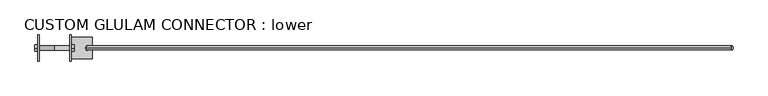
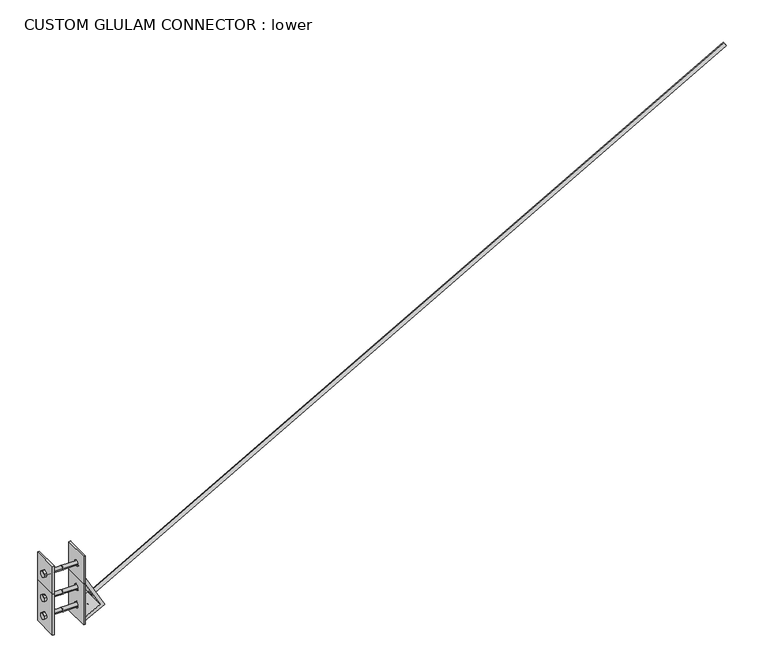
"""IFC4 building model written with IfcOpenShell, lengths in millimetres: fastener geometry, CUSTOM GLULAM CONNECTOR : lower."""

from ifc_helpers import new_model, si_unit, point, frame, frame_2d, origin, place, context, project, spatial, polyline, circle_curve, trimmed, segment, composite_curve, outline, extrude, source, transform, mapped, element, save
from ifc_brep_helpers import plane_surface, revolved_surface, advanced_brep


def custom_glulam_connector_lower_2ef7f48c(model_context):
    return source(origin(), model_context, "Body", "SolidModel", [
        advanced_brep(
        [(-77.7875, -60.325, 211.1375), (-77.7875, -52.3875, 211.1375), (-77.7875, 60.325, 211.1375), (-77.7875, 60.325, 7.9375), (-77.7875, -52.3875, 7.9375), (-77.7875, -60.325, 7.9375), (-77.7875, -13.890625, 160.3375), (-77.7875, 13.890625, 160.3375), (-77.7875, -13.890625, 71.4375), (-77.7875, 13.890625, 71.4375), (-69.85, 13.890625, 160.3375), (-69.85, -13.890625, 160.3375), (-69.85, 13.890625, 71.4375), (-69.85, -13.890625, 71.4375), (-69.85, -60.325, 211.1375), (-69.85, -60.325, 7.9375), (-69.85, 60.325, 7.9375), (-69.85, 60.325, 211.1375)],
        [
            (0, 1),
            (1, 2),
            (2, 3),
            (3, 4),
            (4, 5),
            (5, 0),
            (6, 7, circle_curve(frame((-77.7875, 0.0, 160.3375), z_axis=(1.0, 0.0, 0.0), x_axis=(0.0, -1.0, 0.0)), 13.890625)),
            (7, 6, circle_curve(frame((-77.7875, 0.0, 160.3375), z_axis=(1.0, 0.0, 0.0), x_axis=(0.0, -1.0, 0.0)), 13.890625)),
            (8, 9, circle_curve(frame((-77.7875, 0.0, 71.4375), z_axis=(1.0, 0.0, 0.0), x_axis=(0.0, -1.0, 0.0)), 13.890625)),
            (9, 8, circle_curve(frame((-77.7875, 0.0, 71.4375), z_axis=(1.0, 0.0, 0.0), x_axis=(0.0, -1.0, 0.0)), 13.890625)),
            (10, 7),
            (6, 11),
            (11, 10, circle_curve(frame((-69.85, 0.0, 160.3375), z_axis=(1.0, 0.0, 0.0), x_axis=(0.0, -1.0, 0.0)), 13.890625)),
            (10, 11, circle_curve(frame((-69.85, 0.0, 160.3375), z_axis=(1.0, 0.0, 0.0), x_axis=(0.0, -1.0, 0.0)), 13.890625)),
            (9, 12),
            (12, 13, circle_curve(frame((-69.85, 0.0, 71.4375), z_axis=(1.0, 0.0, 0.0), x_axis=(0.0, -1.0, 0.0)), 13.890625)),
            (13, 8),
            (13, 12, circle_curve(frame((-69.85, 0.0, 71.4375), z_axis=(1.0, 0.0, 0.0), x_axis=(0.0, -1.0, 0.0)), 13.890625)),
            (14, 15),
            (15, 16),
            (16, 17),
            (17, 14),
            (0, 14),
            (17, 2),
            (16, 3),
            (15, 5),
        ],
        [
            plane_surface(frame((-77.7875, 60.325, 211.1375), z_axis=(-1.0, 0.0, 0.0), x_axis=(0.0, 1.0, 0.0))),
            revolved_surface(polyline([(-77.7875, -13.890625, 160.3375), (-69.85, -13.890625, 160.3375)]), (-69.85, 0.0, 160.3375), (-1.0, 0.0, 0.0)),
            revolved_surface(polyline([(-77.7875, -13.890625, 71.4375), (-69.85, -13.890625, 71.4375)]), (-69.85, 0.0, 71.4375), (-1.0, 0.0, 0.0)),
            plane_surface(frame((-69.85, 60.325, 211.1375), z_axis=(1.0, 0.0, 0.0), x_axis=(0.0, -1.0, 0.0))),
            plane_surface(frame((-77.7875, -60.325, 211.1375), z_axis=(0.0, 0.0, 1.0), x_axis=(1.0, 0.0, 0.0))),
            plane_surface(frame((-77.7875, 60.325, 211.1375), z_axis=(0.0, 1.0, 0.0), x_axis=(1.0, 0.0, 0.0))),
            plane_surface(frame((-77.7875, 60.325, 7.9375), z_axis=(0.0, 0.0, -1.0), x_axis=(1.0, 0.0, 0.0))),
            plane_surface(frame((-77.7875, -60.325, 7.9375), z_axis=(0.0, -1.0, 0.0), x_axis=(1.0, 0.0, 0.0))),
        ],
        [
            (0, [[1, 2, 3, 4, 5, 6], [7, 8], [9, 10]]),
            (1, [[11, -7, 12, 13]]),
            (1, [[-11, 14, -12, -8]]),
            (2, [[15, 16, 17, -10]]),
            (2, [[-15, -9, -17, 18]]),
            (3, [[19, 20, 21, 22], [-13, -14], [-18, -16]]),
            (4, [[-2, -1, 23, -22, 24]]),
            (5, [[-3, -24, -21, 25]]),
            (6, [[-5, -4, -25, -20, 26]]),
            (7, [[-6, -26, -19, -23]]),
        ],
    ),
        extrude(outline(polyline([(14.2875, 168.586392), (14.2875, 152.088608), (0.0, 143.8397161), (-14.2875, 152.088608), (-14.2875, 168.586392), (0.0, 176.8352839), (14.2875, 168.586392)])), frame((-90.4875, 0.0, 0.0), z_axis=(1.0, 0.0, 0.0), x_axis=(0.0, 1.0, 0.0)), (0.0, 0.0, 1.0), 12.7),
        extrude(outline(composite_curve([segment(trimmed(circle_curve(frame_2d((0.0, 160.3375)), 9.525), [point((9.525, 160.3375))], [point((-9.525, 160.3375))], False, "CARTESIAN"), True, "CONTINUOUS"), segment(trimmed(circle_curve(frame_2d((0.0, 160.3375)), 9.525), [point((-9.525, 160.3375))], [point((9.525, 160.3375))], False, "CARTESIAN"), True, "CONTINUOUS")], self_intersect=False)), frame((-77.7875, 0.0, 0.0), z_axis=(1.0, 0.0, 0.0), x_axis=(0.0, 1.0, 0.0)), (0.0, 0.0, 1.0), 76.2),
        extrude(outline(polyline([(14.2875, 79.686392), (14.2875, 63.188608), (0.0, 54.9397161), (-14.2875, 63.188608), (-14.2875, 79.686392), (0.0, 87.9352839), (14.2875, 79.686392)])), frame((-90.4875, 0.0, 0.0), z_axis=(1.0, 0.0, 0.0), x_axis=(0.0, 1.0, 0.0)), (0.0, 0.0, 1.0), 12.7),
        extrude(outline(composite_curve([segment(trimmed(circle_curve(frame_2d((0.0, 71.4375)), 9.525), [point((9.525, 71.4375))], [point((-9.525, 71.4375))], False, "CARTESIAN"), True, "CONTINUOUS"), segment(trimmed(circle_curve(frame_2d((0.0, 71.4375)), 9.525), [point((-9.525, 71.4375))], [point((9.525, 71.4375))], False, "CARTESIAN"), True, "CONTINUOUS")], self_intersect=False)), frame((-77.7875, 0.0, 0.0), z_axis=(1.0, 0.0, 0.0), x_axis=(0.0, 1.0, 0.0)), (0.0, 0.0, 1.0), 76.2),
        extrude(outline(polyline([(14.2875, 168.586392), (14.2875, 152.088608), (0.0, 143.8397161), (-14.2875, 152.088608), (-14.2875, 168.586392), (0.0, 176.8352839), (14.2875, 168.586392)])), frame((-90.4875, 0.0, 0.0), z_axis=(1.0, 0.0, 0.0), x_axis=(0.0, 1.0, 0.0)), (0.0, 0.0, 1.0), 12.7),
        extrude(outline(composite_curve([segment(trimmed(circle_curve(frame_2d((0.0, 160.3375)), 9.525), [point((9.525, 160.3375))], [point((-9.525, 160.3375))], False, "CARTESIAN"), True, "CONTINUOUS"), segment(trimmed(circle_curve(frame_2d((0.0, 160.3375)), 9.525), [point((-9.525, 160.3375))], [point((9.525, 160.3375))], False, "CARTESIAN"), True, "CONTINUOUS")], self_intersect=False)), frame((-77.7875, 0.0, 0.0), z_axis=(1.0, 0.0, 0.0), x_axis=(0.0, 1.0, 0.0)), (0.0, 0.0, 1.0), 76.2),
        advanced_brep(
        [(77.7875, -60.325, 211.1375), (77.7875, -60.325, 7.9375), (77.7875, -52.3875, 7.9375), (77.7875, 60.325, 7.9375), (77.7875, 60.325, 211.1375), (77.7875, -52.3875, 211.1375), (77.7875, -13.890625, 71.4375), (77.7875, 13.890625, 71.4375), (77.7875, -13.890625, 160.3375), (77.7875, 13.890625, 160.3375), (69.85, 13.890625, 160.3375), (69.85, -13.890625, 160.3375), (69.85, -13.890625, 71.4375), (69.85, 13.890625, 71.4375), (69.85, -60.325, 211.1375), (69.85, 60.325, 211.1375), (69.85, 60.325, 7.9375), (69.85, -60.325, 7.9375)],
        [
            (0, 1),
            (1, 2),
            (2, 3),
            (3, 4),
            (4, 5),
            (5, 0),
            (6, 7, circle_curve(frame((77.7875, 0.0, 71.4375), z_axis=(-1.0, 0.0, 0.0), x_axis=(0.0, -1.0, 0.0)), 13.890625)),
            (7, 6, circle_curve(frame((77.7875, 0.0, 71.4375), z_axis=(-1.0, 0.0, 0.0), x_axis=(0.0, -1.0, 0.0)), 13.890625)),
            (8, 9, circle_curve(frame((77.7875, 0.0, 160.3375), z_axis=(-1.0, 0.0, 0.0), x_axis=(0.0, -1.0, 0.0)), 13.890625)),
            (9, 8, circle_curve(frame((77.7875, 0.0, 160.3375), z_axis=(-1.0, 0.0, 0.0), x_axis=(0.0, -1.0, 0.0)), 13.890625)),
            (10, 11, circle_curve(frame((69.85, 0.0, 160.3375), z_axis=(-1.0, 0.0, 0.0), x_axis=(0.0, -1.0, 0.0)), 13.890625)),
            (11, 8),
            (9, 10),
            (11, 10, circle_curve(frame((69.85, 0.0, 160.3375), z_axis=(-1.0, 0.0, 0.0), x_axis=(0.0, -1.0, 0.0)), 13.890625)),
            (6, 12),
            (12, 13, circle_curve(frame((69.85, 0.0, 71.4375), z_axis=(-1.0, 0.0, 0.0), x_axis=(0.0, -1.0, 0.0)), 13.890625)),
            (13, 7),
            (13, 12, circle_curve(frame((69.85, 0.0, 71.4375), z_axis=(-1.0, 0.0, 0.0), x_axis=(0.0, -1.0, 0.0)), 13.890625)),
            (14, 15),
            (15, 16),
            (16, 17),
            (17, 14),
            (4, 15),
            (14, 0),
            (3, 16),
            (1, 17),
        ],
        [
            plane_surface(frame((77.7875, 60.325, 211.1375), z_axis=(1.0, 0.0, 0.0), x_axis=(0.0, 1.0, 0.0))),
            revolved_surface(polyline([(77.7875, -13.890625, 160.3375), (69.85, -13.890625, 160.3375)]), (69.85, 0.0, 160.3375), (1.0, 0.0, 0.0)),
            revolved_surface(polyline([(77.7875, -13.890625, 71.4375), (69.85, -13.890625, 71.4375)]), (69.85, 0.0, 71.4375), (1.0, 0.0, 0.0)),
            plane_surface(frame((69.85, 60.325, 211.1375), z_axis=(-1.0, 0.0, 0.0), x_axis=(0.0, -1.0, 0.0))),
            plane_surface(frame((77.7875, -60.325, 211.1375), z_axis=(0.0, 0.0, 1.0), x_axis=(-1.0, 0.0, 0.0))),
            plane_surface(frame((77.7875, 60.325, 211.1375), z_axis=(0.0, 1.0, 0.0), x_axis=(-1.0, 0.0, 0.0))),
            plane_surface(frame((77.7875, 60.325, 7.9375), z_axis=(0.0, 0.0, -1.0), x_axis=(-1.0, 0.0, 0.0))),
            plane_surface(frame((77.7875, -60.325, 7.9375), z_axis=(0.0, -1.0, 0.0), x_axis=(-1.0, 0.0, 0.0))),
        ],
        [
            (0, [[1, 2, 3, 4, 5, 6], [7, 8], [9, 10]]),
            (1, [[11, 12, -10, 13]]),
            (1, [[-9, -12, 14, -13]]),
            (2, [[-7, 15, 16, 17]]),
            (2, [[18, -15, -8, -17]]),
            (3, [[19, 20, 21, 22], [-16, -18], [-14, -11]]),
            (4, [[23, -19, 24, -6, -5]]),
            (5, [[25, -20, -23, -4]]),
            (6, [[26, -21, -25, -3, -2]]),
            (7, [[-24, -22, -26, -1]]),
        ],
    ),
        extrude(outline(polyline([(14.2875, 168.586392), (14.2875, 152.088608), (0.0, 143.8397161), (-14.2875, 152.088608), (-14.2875, 168.586392), (0.0, 176.8352839), (14.2875, 168.586392)])), frame((77.7875, 0.0, 0.0), z_axis=(1.0, 0.0, 0.0), x_axis=(0.0, 1.0, 0.0)), (0.0, 0.0, 1.0), 12.7),
        extrude(outline(composite_curve([segment(trimmed(circle_curve(frame_2d((0.0, 160.3375)), 9.525), [point((9.525, 160.3375))], [point((-9.525, 160.3375))], False, "CARTESIAN"), True, "CONTINUOUS"), segment(trimmed(circle_curve(frame_2d((0.0, 160.3375)), 9.525), [point((-9.525, 160.3375))], [point((9.525, 160.3375))], False, "CARTESIAN"), True, "CONTINUOUS")], self_intersect=False)), frame((1.5875, 0.0, 0.0), z_axis=(1.0, 0.0, 0.0), x_axis=(0.0, 1.0, 0.0)), (0.0, 0.0, 1.0), 76.2),
        extrude(outline(polyline([(14.2875, 79.686392), (14.2875, 63.188608), (0.0, 54.9397161), (-14.2875, 63.188608), (-14.2875, 79.686392), (0.0, 87.9352839), (14.2875, 79.686392)])), frame((77.7875, 0.0, 0.0), z_axis=(1.0, 0.0, 0.0), x_axis=(0.0, 1.0, 0.0)), (0.0, 0.0, 1.0), 12.7),
        extrude(outline(composite_curve([segment(trimmed(circle_curve(frame_2d((0.0, 71.4375)), 9.525), [point((9.525, 71.4375))], [point((-9.525, 71.4375))], False, "CARTESIAN"), True, "CONTINUOUS"), segment(trimmed(circle_curve(frame_2d((0.0, 71.4375)), 9.525), [point((-9.525, 71.4375))], [point((9.525, 71.4375))], False, "CARTESIAN"), True, "CONTINUOUS")], self_intersect=False)), frame((1.5875, 0.0, 0.0), z_axis=(1.0, 0.0, 0.0), x_axis=(0.0, 1.0, 0.0)), (0.0, 0.0, 1.0), 76.2),
        extrude(outline(polyline([(14.2875, 168.586392), (14.2875, 152.088608), (0.0, 143.8397161), (-14.2875, 152.088608), (-14.2875, 168.586392), (0.0, 176.8352839), (14.2875, 168.586392)])), frame((77.7875, 0.0, 0.0), z_axis=(1.0, 0.0, 0.0), x_axis=(0.0, 1.0, 0.0)), (0.0, 0.0, 1.0), 12.7),
        extrude(outline(composite_curve([segment(trimmed(circle_curve(frame_2d((0.0, 160.3375)), 9.525), [point((9.525, 160.3375))], [point((-9.525, 160.3375))], False, "CARTESIAN"), True, "CONTINUOUS"), segment(trimmed(circle_curve(frame_2d((0.0, 160.3375)), 9.525), [point((-9.525, 160.3375))], [point((9.525, 160.3375))], False, "CARTESIAN"), True, "CONTINUOUS")], self_intersect=False)), frame((1.5875, 0.0, 0.0), z_axis=(1.0, 0.0, 0.0), x_axis=(0.0, 1.0, 0.0)), (0.0, 0.0, 1.0), 76.2),
        advanced_brep(
        [(-77.7875, -60.325, 350.8375), (-77.7875, 52.3875, 350.8375), (-77.7875, 60.325, 350.8375), (-77.7875, 60.325, 211.1375), (-77.7875, 52.3875, 211.1375), (-77.7875, -60.325, 211.1375), (-77.7875, -13.890625, 280.9875), (-77.7875, 13.890625, 280.9875), (-69.85, -60.325, 350.8375), (-69.85, -60.325, 211.1375), (-69.85, 60.325, 211.1375), (-69.85, 60.325, 350.8375), (-69.85, 13.890625, 280.9875), (-69.85, -13.890625, 280.9875)],
        [
            (0, 1),
            (1, 2),
            (2, 3),
            (3, 4),
            (4, 5),
            (5, 0),
            (6, 7, circle_curve(frame((-77.7875, 0.0, 280.9875), z_axis=(1.0, 0.0, 0.0), x_axis=(0.0, -1.0, 0.0)), 13.890625)),
            (7, 6, circle_curve(frame((-77.7875, 0.0, 280.9875), z_axis=(1.0, 0.0, 0.0), x_axis=(0.0, -1.0, 0.0)), 13.890625)),
            (8, 9),
            (9, 10),
            (10, 11),
            (11, 8),
            (12, 13, circle_curve(frame((-69.85, 0.0, 280.9875), z_axis=(-1.0, 0.0, 0.0), x_axis=(0.0, -1.0, 0.0)), 13.890625)),
            (13, 12, circle_curve(frame((-69.85, 0.0, 280.9875), z_axis=(-1.0, 0.0, 0.0), x_axis=(0.0, -1.0, 0.0)), 13.890625)),
            (0, 8),
            (11, 2),
            (10, 3),
            (9, 5),
            (12, 7),
            (6, 13),
        ],
        [
            plane_surface(frame((-77.7875, 60.325, 350.8375), z_axis=(-1.0, 0.0, 0.0), x_axis=(0.0, 1.0, 0.0))),
            plane_surface(frame((-69.85, 60.325, 350.8375), z_axis=(1.0, 0.0, 0.0), x_axis=(0.0, -1.0, 0.0))),
            plane_surface(frame((-77.7875, -60.325, 350.8375), z_axis=(0.0, 0.0, 1.0), x_axis=(1.0, 0.0, 0.0))),
            plane_surface(frame((-77.7875, 60.325, 350.8375), z_axis=(0.0, 1.0, 0.0), x_axis=(1.0, 0.0, 0.0))),
            plane_surface(frame((-77.7875, 60.325, 211.1375), z_axis=(0.0, 0.0, -1.0), x_axis=(1.0, 0.0, 0.0))),
            plane_surface(frame((-77.7875, -60.325, 211.1375), z_axis=(0.0, -1.0, 0.0), x_axis=(1.0, 0.0, 0.0))),
            revolved_surface(polyline([(-77.7875, -13.890625, 280.9875), (-69.85, -13.890625, 280.9875)]), (-69.85, 0.0, 280.9875), (-1.0, 0.0, 0.0)),
        ],
        [
            (0, [[1, 2, 3, 4, 5, 6], [7, 8]]),
            (1, [[9, 10, 11, 12], [13, 14]]),
            (2, [[-2, -1, 15, -12, 16]]),
            (3, [[-3, -16, -11, 17]]),
            (4, [[-5, -4, -17, -10, 18]]),
            (5, [[-6, -18, -9, -15]]),
            (6, [[19, -7, 20, -13]]),
            (6, [[-19, -14, -20, -8]]),
        ],
    ),
        extrude(outline(polyline([(14.2875, 289.236392), (14.2875, 272.738608), (0.0, 264.4897161), (-14.2875, 272.738608), (-14.2875, 289.236392), (0.0, 297.4852839), (14.2875, 289.236392)])), frame((-90.4875, 0.0, 0.0), z_axis=(1.0, 0.0, 0.0), x_axis=(0.0, 1.0, 0.0)), (0.0, 0.0, 1.0), 12.7),
        extrude(outline(composite_curve([segment(trimmed(circle_curve(frame_2d((0.0, 280.9875)), 9.525), [point((9.525, 280.9875))], [point((-9.525, 280.9875))], False, "CARTESIAN"), True, "CONTINUOUS"), segment(trimmed(circle_curve(frame_2d((0.0, 280.9875)), 9.525), [point((-9.525, 280.9875))], [point((9.525, 280.9875))], False, "CARTESIAN"), True, "CONTINUOUS")], self_intersect=False)), frame((-77.7875, 0.0, 0.0), z_axis=(1.0, 0.0, 0.0), x_axis=(0.0, 1.0, 0.0)), (0.0, 0.0, 1.0), 76.2),
        advanced_brep(
        [(77.7875, -60.325, 350.8375), (77.7875, -60.325, 211.1375), (77.7875, 52.3875, 211.1375), (77.7875, 60.325, 211.1375), (77.7875, 60.325, 350.8375), (77.7875, 52.3875, 350.8375), (77.7875, -13.890625, 280.9875), (77.7875, 13.890625, 280.9875), (69.85, -60.325, 350.8375), (69.85, 60.325, 350.8375), (69.85, 60.325, 211.1375), (69.85, -60.325, 211.1375), (69.85, 13.890625, 280.9875), (69.85, -13.890625, 280.9875)],
        [
            (0, 1),
            (1, 2),
            (2, 3),
            (3, 4),
            (4, 5),
            (5, 0),
            (6, 7, circle_curve(frame((77.7875, 0.0, 280.9875), z_axis=(-1.0, 0.0, 0.0), x_axis=(0.0, -1.0, 0.0)), 13.890625)),
            (7, 6, circle_curve(frame((77.7875, 0.0, 280.9875), z_axis=(-1.0, 0.0, 0.0), x_axis=(0.0, -1.0, 0.0)), 13.890625)),
            (8, 9),
            (9, 10),
            (10, 11),
            (11, 8),
            (12, 13, circle_curve(frame((69.85, 0.0, 280.9875), z_axis=(1.0, 0.0, 0.0), x_axis=(0.0, -1.0, 0.0)), 13.890625)),
            (13, 12, circle_curve(frame((69.85, 0.0, 280.9875), z_axis=(1.0, 0.0, 0.0), x_axis=(0.0, -1.0, 0.0)), 13.890625)),
            (4, 9),
            (8, 0),
            (3, 10),
            (1, 11),
            (13, 6),
            (7, 12),
        ],
        [
            plane_surface(frame((77.7875, 60.325, 350.8375), z_axis=(1.0, 0.0, 0.0), x_axis=(0.0, 1.0, 0.0))),
            plane_surface(frame((69.85, 60.325, 350.8375), z_axis=(-1.0, 0.0, 0.0), x_axis=(0.0, -1.0, 0.0))),
            plane_surface(frame((77.7875, -60.325, 350.8375), z_axis=(0.0, 0.0, 1.0), x_axis=(-1.0, 0.0, 0.0))),
            plane_surface(frame((77.7875, 60.325, 350.8375), z_axis=(0.0, 1.0, 0.0), x_axis=(-1.0, 0.0, 0.0))),
            plane_surface(frame((77.7875, 60.325, 211.1375), z_axis=(0.0, 0.0, -1.0), x_axis=(-1.0, 0.0, 0.0))),
            plane_surface(frame((77.7875, -60.325, 211.1375), z_axis=(0.0, -1.0, 0.0), x_axis=(-1.0, 0.0, 0.0))),
            revolved_surface(polyline([(77.7875, -13.890625, 280.9875), (69.85, -13.890625, 280.9875)]), (69.85, 0.0, 280.9875), (1.0, 0.0, 0.0)),
        ],
        [
            (0, [[1, 2, 3, 4, 5, 6], [7, 8]]),
            (1, [[9, 10, 11, 12], [13, 14]]),
            (2, [[15, -9, 16, -6, -5]]),
            (3, [[17, -10, -15, -4]]),
            (4, [[18, -11, -17, -3, -2]]),
            (5, [[-16, -12, -18, -1]]),
            (6, [[-14, 19, -8, 20]]),
            (6, [[-7, -19, -13, -20]]),
        ],
    ),
        extrude(outline(polyline([(14.2875, 289.236392), (14.2875, 272.738608), (0.0, 264.4897161), (-14.2875, 272.738608), (-14.2875, 289.236392), (0.0, 297.4852839), (14.2875, 289.236392)])), frame((77.7875, 0.0, 0.0), z_axis=(1.0, 0.0, 0.0), x_axis=(0.0, 1.0, 0.0)), (0.0, 0.0, 1.0), 12.7),
        extrude(outline(composite_curve([segment(trimmed(circle_curve(frame_2d((0.0, 280.9875)), 9.525), [point((9.525, 280.9875))], [point((-9.525, 280.9875))], False, "CARTESIAN"), True, "CONTINUOUS"), segment(trimmed(circle_curve(frame_2d((0.0, 280.9875)), 9.525), [point((-9.525, 280.9875))], [point((9.525, 280.9875))], False, "CARTESIAN"), True, "CONTINUOUS")], self_intersect=False)), frame((1.5875, 0.0, 0.0), z_axis=(1.0, 0.0, 0.0), x_axis=(0.0, 1.0, 0.0)), (0.0, 0.0, 1.0), 76.2),
        extrude(outline(composite_curve([segment(trimmed(circle_curve(frame_2d((0.0, 9.525)), 9.525), [point((0.0, 19.05))], [point((0.0, 0.0))], False, "CARTESIAN"), True, "CONTINUOUS"), segment(trimmed(circle_curve(frame_2d((0.0, 9.525)), 9.525), [point((0.0, 0.0))], [point((0.0, 19.05))], False, "CARTESIAN"), True, "CONTINUOUS")], self_intersect=False)), frame((155.1212692, 0.0, 104.8231986), z_axis=(0.8703556959399006, 0.0, 0.4924235601034656), x_axis=(0.0, 1.0, 0.0)), (0.0, 0.0, 1.0), 3429.0),
        advanced_brep(
        [(175.4460516, 50.8, 68.8992672), (77.7875, 50.8, 15.875), (77.7875, 50.8, 33.9390543), (153.67429, 50.8, 75.1422194), (77.7875, 50.8, 209.2716667), (77.7875, 50.8, 241.5101729), (175.4460516, -50.8, 68.8992672), (77.7875, -50.8, 241.5101729), (77.7875, -50.8, 209.2716667), (153.67429, -50.8, 75.1422194), (77.7875, -50.8, 33.9390543), (77.7875, -50.8, 15.875), (155.707561, 0.0, 103.7869313), (145.1543086, 0.0, 122.4397418), (131.3374119, 0.0, 114.6225178), (141.8906643, 0.0, 95.9697073), (123.5760275, 0.0, 58.8001963), (122.8784665, 0.0, 58.4214515), (130.4533618, 0.0, 44.4702298), (131.1509229, 0.0, 44.8489746)],
        [
            (0, 1),
            (1, 2),
            (2, 3),
            (3, 4),
            (4, 5),
            (5, 0),
            (6, 7),
            (7, 8),
            (8, 9),
            (9, 10),
            (10, 11),
            (11, 6),
            (5, 7),
            (6, 0),
            (12, 13, circle_curve(frame((150.4309348, 0.0, 113.1133366), z_axis=(-0.8703556959399006, 0.0, -0.4924235601034656), x_axis=(-0.4924235601034656, 0.0, 0.8703556959399006)), 10.715625)),
            (13, 12, circle_curve(frame((150.4309348, 0.0, 113.1133366), z_axis=(-0.8703556959399006, 0.0, -0.4924235601034656), x_axis=(-0.4924235601034656, 0.0, 0.8703556959399006)), 10.715625)),
            (4, 8),
            (3, 9),
            (14, 15, circle_curve(frame((136.6140381, 0.0, 105.2961126), z_axis=(0.8703556959399006, 0.0, 0.4924235601034656), x_axis=(-0.4924235601034656, 0.0, 0.8703556959399006)), 10.715625)),
            (15, 14, circle_curve(frame((136.6140381, 0.0, 105.2961126), z_axis=(0.8703556959399006, 0.0, 0.4924235601034656), x_axis=(-0.4924235601034656, 0.0, 0.8703556959399006)), 10.715625)),
            (2, 10),
            (16, 17, circle_curve(frame((123.227247, 0.0, 58.6108239), z_axis=(0.47715876025960574, 0.0, -0.8788171126619669), x_axis=(0.8788171126619669, 0.0, 0.47715876025960574)), 0.396875)),
            (17, 16, circle_curve(frame((123.227247, 0.0, 58.6108239), z_axis=(0.47715876025960574, 0.0, -0.8788171126619669), x_axis=(0.8788171126619669, 0.0, 0.47715876025960574)), 0.396875)),
            (1, 11),
            (18, 19, circle_curve(frame((130.8021423, 0.0, 44.6596022), z_axis=(-0.47715876025960574, 0.0, 0.8788171126619669), x_axis=(0.8788171126619669, 0.0, 0.47715876025960574)), 0.396875)),
            (19, 18, circle_curve(frame((130.8021423, 0.0, 44.6596022), z_axis=(-0.47715876025960574, 0.0, 0.8788171126619669), x_axis=(0.8788171126619669, 0.0, 0.47715876025960574)), 0.396875)),
            (13, 14),
            (15, 12),
            (19, 16),
            (17, 18),
        ],
        [
            plane_surface(frame((77.7875, 50.8, 241.5101729), z_axis=(0.0, 1.0, 0.0), x_axis=(-0.4924235601034656, 0.0, 0.8703556959399006))),
            plane_surface(frame((77.7875, -50.8, 241.5101729), z_axis=(0.0, -1.0, 0.0), x_axis=(0.4924235601034656, 0.0, -0.8703556959399006))),
            plane_surface(frame((175.4460516, 50.8, 68.8992672), z_axis=(0.8703556959399006, 0.0, 0.4924235601034656), x_axis=(0.0, -1.0, 0.0))),
            plane_surface(frame((77.7875, 50.8, 241.5101729), z_axis=(-1.0, 0.0, 0.0), x_axis=(0.0, -1.0, 0.0))),
            plane_surface(frame((77.7875, 50.8, 209.2716667), z_axis=(-0.8703556959399004, 0.0, -0.49242356010346605), x_axis=(0.0, -1.0, 0.0))),
            plane_surface(frame((153.67429, 50.8, 75.1422194), z_axis=(-0.4771587602596049, 0.0, 0.8788171126619673), x_axis=(0.0, -1.0, 0.0))),
            plane_surface(frame((77.7875, 50.8, 33.9390543), z_axis=(-1.0, 0.0, 0.0), x_axis=(0.0, -1.0, 0.0))),
            plane_surface(frame((77.7875, 50.8, 15.875), z_axis=(0.47715876025960613, 0.0, -0.8788171126619666), x_axis=(0.0, -1.0, 0.0))),
            revolved_surface(polyline([(131.33741187434143, 0.0, 114.62251781425239), (145.1543085887663, 0.0, 122.43974185430599)]), (150.4309348, 0.0, 113.1133366), (-0.8703556959399006, 0.0, -0.4924235601034656)),
            revolved_surface(polyline([(123.57602749491133, 0.0, 58.80019629723708), (131.15092285819438, 0.0, 44.848974552392434)]), (130.8021423, 0.0, 44.6596022), (-0.47715876025960574, 0.0, 0.8788171126619669)),
        ],
        [
            (0, [[1, 2, 3, 4, 5, 6]]),
            (1, [[7, 8, 9, 10, 11, 12]]),
            (2, [[13, -7, 14, -6], [15, 16]]),
            (3, [[17, -8, -13, -5]]),
            (4, [[18, -9, -17, -4], [19, 20]]),
            (5, [[21, -10, -18, -3], [22, 23]]),
            (6, [[24, -11, -21, -2]]),
            (7, [[-14, -12, -24, -1], [25, 26]]),
            (8, [[-16, 27, -20, 28]]),
            (8, [[-19, -27, -15, -28]]),
            (9, [[-26, 29, -23, 30]]),
            (9, [[-22, -29, -25, -30]]),
        ],
    ),
    ])


if __name__ == "__main__":
    model = new_model("IFC4")
    model_context = context("Model", 3, world=origin())
    ifc_project = project(units=[si_unit("LENGTHUNIT", "METRE", prefix="MILLI")], contexts=[model_context])
    site = spatial("IfcSite", under=ifc_project)
    building = spatial("IfcBuilding", under=site)
    placement = place(None, origin())
    custom_glulam_connector_lower_shape = custom_glulam_connector_lower_2ef7f48c(model_context)
    element("IfcFastener", 1, ObjectType="CUSTOM GLULAM CONNECTOR : lower", at=placement, inside=building, context=model_context, shape_type="MappedRepresentation", body=[
        mapped(custom_glulam_connector_lower_shape, transform((0.0, 0.0, 0.0), x_axis=(1.0, 0.0, 0.0), y_axis=(0.0, 1.0, 0.0), z_axis=(0.0, 0.0, 1.0))),
    ])
    save(model, "model.ifc")

# Revit data of these elements
# Type "CUSTOM GLULAM CONNECTOR : lower"
#   Width - Top = 0' - 5 1/2"
#   Top/Bottom Plate Thickness = 0' - 0 5/16"
#   Top/Bottom Plate - Width = 0' - 7 1/2"
#   Rod Radius = 0' - 0 3/8"
#   Rod Length [instance default] = 11' - 4"
#   Plate Thickness = 0' - 0 5/16"
#   Offset - Upper Plate 2 = 0' - 0"
#   Height of Plate = 0' - 8"
#   Width - Bottom = 0' - 5 1/2"
#   Plate Width = 0' - 4 3/4"
#   Bracket Width = 0' - 4"
#   Bracket Thickness = 0' - 0 5/8"
#   Bracket Offset in X = 0' - 3 1/16"
#   Bracket Offset in Y = 0' - 0 3/8"
#   Bracket Offset = 0' - 0 5/8"
#   Bracket Leg = 0' - 4 3/8"
#   Bracket Hole Radius - Up = 0' - 0 27/64"
#   Bracket Hole Radius - Down = 0' - 0 1/64"
#   Bracket Hole Offset = 0' - 2"
#   Beam Width = 0' - 7 3/8"
#   Angle 2 = 29.50°
#   Angle 1 = 118.50°
#   Top Plate Visible = no
#   Rod Visibility = yes
#   Plate Visibility - Upper Right 2 = no
#   Plate Visibility - Upper Right 1 = yes
#   Plate Visibility - Upper Left 2 = no
#   Plate Visibility - Upper Left 1 = yes
#   Plate Visibility - Lower Right 2 = no
#   Plate Visibility - Lower Right 1 = yes
#   Plate Visibility - Lower Left 2 = no
#   Plate Visibility - Lower Left 1 = yes
#   Bracket Visibility = yes
#   Bottom Plate Visible = no
#   Upper Plates - 2 = element 1407869
#   Upper Plates - 1 = element 1407869
#   Lower Plates = element 1407870
#   Bracket Material = 5/8" STEEL ANGLE (HDG AFTER FABRICATION)
#   URL = ""
# Element 1 (IfcFastener, "CUSTOM GLULAM CONNECTOR : lower")
#   Rod Length = 11' - 3"
#   Materials on its faces: "3/4\" LAG BOLT (THRU BOLT IF PLATE ON OPP. SIDE OF STRUCT MEMBER)", "5/16\" STEEL PLATE (HDG AFTER FABRICATION)", "5/8\" STEEL ANGLE (HDG AFTER FABRICATION)", "3/4\" STEEL ROD (THREADED AT ENDS) - W/ TURN BUCKLE"
# Materials
#   "5/8\" STEEL ANGLE (HDG AFTER FABRICATION)": class "Generic", colour RGB 195 195 195, transparency 0, Cost = 0
#   "3/4\" LAG BOLT (THRU BOLT IF PLATE ON OPP. SIDE OF STRUCT MEMBER)": class "Generic", colour RGB 120 120 120, transparency 0, Cost = 0
#   "5/16\" STEEL PLATE (HDG AFTER FABRICATION)": class "Generic", colour RGB 232 232 232, transparency 0, Cost = 0
#   "3/4\" STEEL ROD (THREADED AT ENDS) - W/ TURN BUCKLE": class "Generic", colour RGB 120 120 120, transparency 0, Cost = 0
